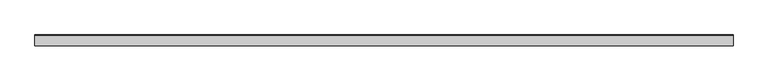
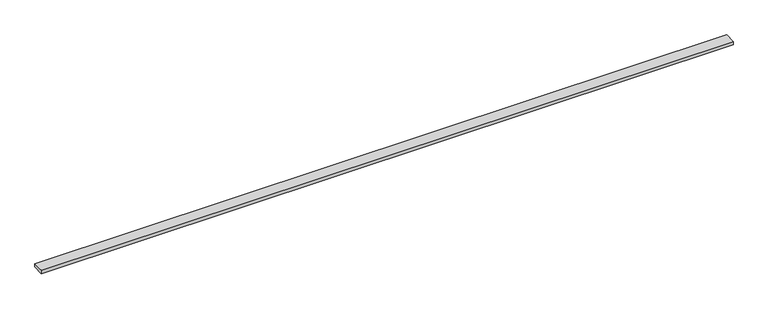
"""IFC4 building model written with IfcOpenShell, lengths in millimetres: proxy geometry, Inner panel:Inner panel:1:Inner panel:1 : Inner panel:Inner panel:300324:2:Inner panel:1:Inner panel:1 : Inner panel:Inner panel:300324:2 : Inner panel:Inner panel:1:Inner panel:1 : Inner panel:Inner panel:300324:300043:18 : Inner panel:Inner panel:1:Inner panel:1 : Inner panel:Inner panel:300324:2:Inner panel:1:Inner panel:1 : Inner panel:Inner panel:300324:2 : Inner panel:Inner panel:1:Inner panel:1 : Inner panel:Inner panel:300324:300043:308120."""

from ifc_helpers import new_model, si_unit, frame, origin, place, context, project, spatial, polyline, outline, extrude, source, transform, mapped, element, save


def generic_models_5f386680(model_context):
    return source(origin(), model_context, "Body", "SweptSolid", [
        extrude(outline(polyline([(0.0, -75.8934962), (0.0, 0.0), (4876.8, 0.0), (4876.8, -75.8934962), (0.0, -75.8934962)])), frame((596182.8367239, -568407.8188757, 4365.8460002), z_axis=(0.0, -0.04163054471215047, 0.9991330730923532), x_axis=(-1.0, 0.0, 0.0)), (0.0, 0.0, 1.0), 25.4),
    ])


if __name__ == "__main__":
    model = new_model("IFC4")
    model_context = context("Model", 3, world=origin())
    ifc_project = project(units=[si_unit("LENGTHUNIT", "METRE", prefix="MILLI")], contexts=[model_context])
    site = spatial("IfcSite", under=ifc_project)
    building = spatial("IfcBuilding", under=site)
    placement = place(None, origin())
    generic_models_shape = generic_models_5f386680(model_context)
    element("IfcBuildingElementProxy", 1, Name="Inner panel:Inner panel:1:Inner panel:1 : Inner panel:Inner panel:300324:2:Inner panel:1:Inner panel:1 : Inner panel:Inner panel:300324:2 : Inner panel:Inner panel:1:Inner panel:1 : Inner panel:Inner panel:300324:300043:18 : Inner panel:Inner panel:1:Inner panel:1 : Inner panel:Inner panel:300324:2:Inner panel:1:Inner panel:1 : Inner panel:Inner panel:300324:2 : Inner panel:Inner panel:1:Inner panel:1 : Inner panel:Inner panel:300324:300043:308120", ObjectType="Inner panel:Inner panel:1:Inner panel:1 : Inner panel:Inner panel:300324:2:Inner panel:1:Inner panel:1 : Inner panel:Inner panel:300324:2 : Inner panel:Inner panel:1:Inner panel:1 : Inner panel:Inner panel:300324:300043:18 : Inner panel:Inner panel:1:Inner panel:1 : Inner panel:Inner panel:300324:2:Inner panel:1:Inner panel:1 : Inner panel:Inner panel:300324:2 : Inner panel:Inner panel:1:Inner panel:1 : Inner panel:Inner panel:300324:300043:308120", at=placement, inside=building, context=model_context, shape_type="MappedRepresentation", body=[
        mapped(generic_models_shape, transform((0.0, 0.0, 0.0), x_axis=(1.0, 0.0, 0.0), y_axis=(0.0, 1.0, 0.0), z_axis=(0.0, 0.0, 1.0))),
    ])
    save(model, "model.ifc")

# Revit data of these elements
# Type "Inner panel:Inner panel:1:Inner panel:1 : Inner panel:Inner panel:300324:2:Inner panel:1:Inner panel:1 : Inner panel:Inner panel:300324:2 : Inner panel:Inner panel:1:Inner panel:1 : Inner panel:Inner panel:300324:300043:18 : Inner panel:Inner panel:1:Inner panel:1 : Inner panel:Inner panel:300324:2:Inner panel:1:Inner panel:1 : Inner panel:Inner panel:300324:2 : Inner panel:Inner panel:1:Inner panel:1 : Inner panel:Inner panel:300324:300043:308120"
#   NameOverride = "Inner panel:Inner panel:1:Inner panel:1 : Inner panel:Inner panel:300324:2:Inner panel:1:Inner panel:1 : Inner panel:Inner panel:300324:2 : Inner panel:Inner panel:1:Inner panel:1 : Inner panel:Inner panel:300324:300043:308120"
#   ObjectTypeOverride = "Inner panel:1:Inner panel:1 : Inner panel:Inner panel:300324:2 : Inner panel:Inner panel:1:Inner panel:1 : Inner panel:Inner panel:300324:300043"
#   Reference = "Inner panel"
#   Tag = "308120"
# Element 1 (IfcBuildingElementProxy, "Inner panel:Inner panel:1:Inner panel:1 : Inner panel:Inner panel:300324:2:Inner panel:1:Inner panel:1 : Inner panel:Inner panel:300324:2 : Inner panel:Inner panel:1:Inner panel:1 : Inner panel:Inner panel:300324:300043:18 : Inner panel:Inner panel:1:Inner panel:1 : Inner panel:Inner panel:300324:2:Inner panel:1:Inner panel:1 : Inner panel:Inner panel:300324:2 : Inner panel:Inner panel:1:Inner panel:1 : Inner panel:Inner panel:300324:300043:308120")
#   Materials on its faces: "1\" THERMAL SPACER @ PURLIN"
# Materials
#   "1\" THERMAL SPACER @ PURLIN": class "Unassigned", colour RGB 205 188 106, transparency 0, Cost = 0
